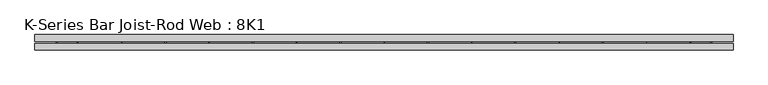
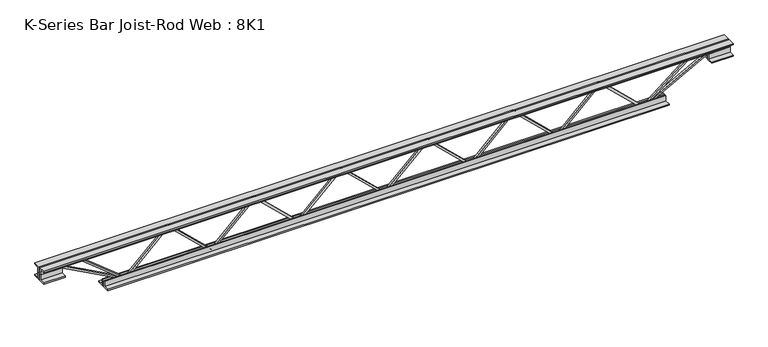
"""IFC4 building model written with IfcOpenShell, lengths in millimetres: beam geometry, K-Series Bar Joist-Rod Web : 8K1."""

import ifcopenshell
import ifcopenshell.guid

model = None  # the IFC model being written
_history = None  # IfcOwnerHistory: only IFC2X3 demands one
_inside = {}  # id of a spatial element -> (the spatial element, [elements in it])
_under = {}  # id of a project, library or spatial element -> (it, [spatial elements below it])
_declared = {}  # id of a project -> (the project, [libraries it declares])
_typed = {}  # id of a type object -> (the type object, [elements of that type])
_made_of = {}  # id of a material, layer set ... -> (it, [elements and type objects made of it])


def new_model(schema):
    """Start an empty IFC model of exactly this schema.

    Asked for "IFC4X3", IfcOpenShell would pick the latest addendum, in which some entities
    have other attributes; the version numbers below select the first issue.
    IFC2X3 requires an IfcOwnerHistory on every rooted entity: one is made here for all.
    """
    global model, _history
    if schema == "IFC4X3":
        model = ifcopenshell.file(schema_version=(4, 3, 0, 0))
    else:
        model = ifcopenshell.file(schema=schema)
    _inside.clear()
    _under.clear()
    _declared.clear()
    _typed.clear()
    _made_of.clear()
    _history = None
    if model.schema == "IFC2X3":
        org = make("IfcOrganization", Name="unknown")
        user = make(
            "IfcPersonAndOrganization",
            ThePerson=make("IfcPerson", FamilyName="unknown"),
            TheOrganization=org,
        )
        app = make(
            "IfcApplication",
            ApplicationDeveloper=org,
            Version="unknown",
            ApplicationFullName="unknown",
            ApplicationIdentifier="unknown",
        )
        _history = make(
            "IfcOwnerHistory",
            OwningUser=user,
            OwningApplication=app,
            ChangeAction="ADDED",
            CreationDate=0,
        )
    return model


def make(cls, **values):
    """One entity of the class cls with the attributes given. An attribute that is None is left unset."""
    return model.create_entity(
        cls, **{name: value for name, value in values.items() if value is not None}
    )


def rooted(cls, **values):
    """An entity with a GlobalId (a new one), such as an element, a storey or a relation."""
    return make(cls, GlobalId=ifcopenshell.guid.new(), OwnerHistory=_history, **values)


def si_unit(unit_type, name, prefix=None):
    """IfcSIUnit, for example si_unit("LENGTHUNIT", "METRE", prefix="MILLI")."""
    return make("IfcSIUnit", UnitType=unit_type, Prefix=prefix, Name=name)


def assignment(units):
    """IfcUnitAssignment: the units of a project."""
    return None if units is None else make("IfcUnitAssignment", Units=units)


def point(xyz):
    """IfcCartesianPoint."""
    return None if xyz is None else make("IfcCartesianPoint", Coordinates=xyz)


def direction(xyz):
    """IfcDirection."""
    return None if xyz is None else make("IfcDirection", DirectionRatios=xyz)


def frame(location, z_axis=None, x_axis=None):
    """IfcAxis2Placement3D, a coordinate frame: its origin and axes. An axis left out is left unset."""
    return make(
        "IfcAxis2Placement3D",
        Location=point(location),
        Axis=direction(z_axis),
        RefDirection=direction(x_axis),
    )


def origin():
    """The frame at (0, 0, 0) with its axes left unset."""
    return frame((0.0, 0.0, 0.0))


def place(relative_to, where):
    """IfcLocalPlacement: puts the frame where relative to a parent placement (None: the world)."""
    return make(
        "IfcLocalPlacement", PlacementRelTo=relative_to, RelativePlacement=where
    )


def context(
    kind, dimensions, precision=None, world=None, true_north=None, identifier=None
):
    """IfcGeometricRepresentationContext, for example the 3D "Model" context."""
    return make(
        "IfcGeometricRepresentationContext",
        ContextIdentifier=identifier,
        ContextType=kind,
        CoordinateSpaceDimension=dimensions,
        Precision=precision,
        WorldCoordinateSystem=world,
        TrueNorth=true_north,
    )


def project(units=None, contexts=None):
    """IfcProject with its units and contexts."""
    return rooted(
        "IfcProject",
        Name="project",
        RepresentationContexts=contexts,
        UnitsInContext=assignment(units),
    )


def spatial(cls, under=None, at=None, **own):
    """A site, building, storey or space (cls), placed at a placement, below another one or the project."""
    s = rooted(cls, ObjectPlacement=at, **own)
    if under is not None:
        _under.setdefault(under.id(), (under, []))[1].append(s)
    return s


def polyline(points):
    """IfcPolyline through the points."""
    return make("IfcPolyline", Points=[point(p) for p in points])


def outline(outer, holes=None, kind="AREA"):
    """IfcArbitraryClosedProfileDef: a profile drawn as a closed curve; with holes, ...WithVoids."""
    if holes is None:
        return make("IfcArbitraryClosedProfileDef", ProfileType=kind, OuterCurve=outer)
    return make(
        "IfcArbitraryProfileDefWithVoids",
        ProfileType=kind,
        OuterCurve=outer,
        InnerCurves=holes,
    )


def extrude(swept, where, along, depth):
    """IfcExtrudedAreaSolid: the profile swept, set in the frame where, extruded along a direction by depth."""
    return make(
        "IfcExtrudedAreaSolid",
        SweptArea=swept,
        Position=where,
        ExtrudedDirection=direction(along),
        Depth=depth,
    )


def shape(context_of_items, identifier, shape_type, items):
    """IfcShapeRepresentation: the items that make up one representation, for example the "Body"."""
    return make(
        "IfcShapeRepresentation",
        ContextOfItems=context_of_items,
        RepresentationIdentifier=identifier,
        RepresentationType=shape_type,
        Items=items,
    )


def source(mapping_origin, context_of_items, identifier, shape_type, items):
    """IfcRepresentationMap: a shape defined once, which mapped items show again and again."""
    return make(
        "IfcRepresentationMap",
        MappingOrigin=mapping_origin,
        MappedRepresentation=shape(context_of_items, identifier, shape_type, items),
    )


def transform(
    local_origin,
    x_axis=None,
    y_axis=None,
    z_axis=None,
    scale=None,
    scale2=None,
    scale3=None,
    uniform=True,
):
    """IfcCartesianTransformationOperator3D, or its non-uniform kind. x_axis, y_axis, z_axis: its Axis1, 2, 3."""
    if uniform:
        return make(
            "IfcCartesianTransformationOperator3D",
            Axis1=direction(x_axis),
            Axis2=direction(y_axis),
            LocalOrigin=point(local_origin),
            Scale=scale,
            Axis3=direction(z_axis),
        )
    return make(
        "IfcCartesianTransformationOperator3DnonUniform",
        Axis1=direction(x_axis),
        Axis2=direction(y_axis),
        LocalOrigin=point(local_origin),
        Scale=scale,
        Axis3=direction(z_axis),
        Scale2=scale2,
        Scale3=scale3,
    )


def mapped(mapping_source, mapping_target):
    """IfcMappedItem: shows the shape of a source again, moved by a transform."""
    return make(
        "IfcMappedItem", MappingSource=mapping_source, MappingTarget=mapping_target
    )


def made_of(thing, what):
    """Note that an element or type object is made of a material, layer set ...; save() writes the relation."""
    if what is not None:
        _made_of.setdefault(what.id(), (what, []))[1].append(thing)
    return thing


def element(
    cls,
    number,
    at=None,
    inside=None,
    cuts=None,
    type_object=None,
    material=None,
    context=None,
    identifier="Body",
    shape_type=None,
    held_by="IfcProductDefinitionShape",
    body=None,
    shapes=None,
    **own,
):
    """One element of the class cls, such as IfcWall. Its Tag is "e" and its number.

    at: its placement. inside: the storey or other place that contains it. cuts: it is an
    opening in that element (IfcRelVoidsElement). A single representation is given by context,
    identifier, shape_type and body (its items); several are given by shapes. held_by: the class
    of the entity that holds the representations. save() writes the other relations.
    """
    e = rooted(cls, Tag="e%d" % number, ObjectPlacement=at, **own)
    if body is not None:
        shapes = [shape(context, identifier, shape_type, body)]
    if shapes is not None:
        e.Representation = make(held_by, Representations=shapes)
    if inside is not None:
        _inside.setdefault(inside.id(), (inside, []))[1].append(e)
    if cuts is not None:
        rooted(
            "IfcRelVoidsElement", RelatingBuildingElement=cuts, RelatedOpeningElement=e
        )
    if type_object is not None:
        _typed.setdefault(type_object.id(), (type_object, []))[1].append(e)
    return made_of(e, material)


def aggregate(whole, parts):
    """IfcRelAggregates: a whole, such as a stair, and the parts it consists of."""
    return rooted("IfcRelAggregates", RelatingObject=whole, RelatedObjects=parts)


def save(model, path):
    """Write the relations noted so far, then the file.

    IfcRelAggregates (storeys below a building ...), IfcRelContainedInSpatialStructure (elements
    in a storey), IfcRelDefinesByType, IfcRelAssociatesMaterial and IfcRelDeclares: one each for
    every whole, place, type object, material and project.
    """
    for whole, parts in _under.values():
        aggregate(whole, parts)
    for where, things in _inside.values():
        rooted(
            "IfcRelContainedInSpatialStructure",
            RelatedElements=things,
            RelatingStructure=where,
        )
    for kind, things in _typed.values():
        rooted("IfcRelDefinesByType", RelatedObjects=things, RelatingType=kind)
    for what, things in _made_of.values():
        rooted("IfcRelAssociatesMaterial", RelatedObjects=things, RelatingMaterial=what)
    for by, libraries in _declared.values():
        rooted("IfcRelDeclares", RelatingContext=by, RelatedDefinitions=libraries)
    model.write(path)


def k_series_bar_joist_rod_web_8k1_5ba47054(model_context):
    return source(origin(), model_context, "Body", "SweptSolid", [
        extrude(outline(polyline([(-90.4875, 411.0474986), (-100.0125, 411.0474986), (-100.0125, 416.133385), (90.4875, 615.3071343), (90.4875, 617.8353616), (-100.0125, 817.0091109), (-100.0125, 822.0949973), (-90.4875, 822.0949973), (-90.4875, 820.8308836), (100.0125, 621.6571343), (100.0125, 611.4853616), (-90.4875, 412.3116123), (-90.4875, 411.0474986)])), frame((0.0, -4.7625, 0.0), z_axis=(0.0, 1.0, 0.0), x_axis=(0.0, 0.0, 1.0)), (0.0, 0.0, 1.0), 9.525),
        extrude(outline(polyline([(-90.4875, 0.0), (-100.0125, 0.0), (-100.0125, 5.0858863), (90.4875, 204.2596356), (90.4875, 206.787863), (-100.0125, 405.9616123), (-100.0125, 411.0474986), (-90.4875, 411.0474986), (-90.4875, 409.783385), (100.0125, 210.6096356), (100.0125, 200.437863), (-90.4875, 1.2641137), (-90.4875, 0.0)])), frame((0.0, -4.7625, 0.0), z_axis=(0.0, 1.0, 0.0), x_axis=(0.0, 0.0, 1.0)), (0.0, 0.0, 1.0), 9.525),
        extrude(outline(polyline([(-90.4875, -411.0474986), (-100.0125, -411.0474986), (-100.0125, -405.9616123), (90.4875, -206.787863), (90.4875, -204.2596356), (-100.0125, -5.0858863), (-100.0125, 0.0), (-90.4875, 0.0), (-90.4875, -1.2641137), (100.0125, -200.437863), (100.0125, -210.6096356), (-90.4875, -409.783385), (-90.4875, -411.0474986)])), frame((0.0, -4.7625, 0.0), z_axis=(0.0, 1.0, 0.0), x_axis=(0.0, 0.0, 1.0)), (0.0, 0.0, 1.0), 9.525),
        extrude(outline(polyline([(-90.4875, -822.0949973), (-100.0125, -822.0949973), (-100.0125, -817.0091109), (90.4875, -617.8353616), (90.4875, -615.3071343), (-100.0125, -416.133385), (-100.0125, -411.0474986), (-90.4875, -411.0474986), (-90.4875, -412.3116123), (100.0125, -611.4853616), (100.0125, -621.6571343), (-90.4875, -820.8308836), (-90.4875, -822.0949973)])), frame((0.0, -4.7625, 0.0), z_axis=(0.0, 1.0, 0.0), x_axis=(0.0, 0.0, 1.0)), (0.0, 0.0, 1.0), 9.525),
        extrude(outline(polyline([(-90.4875, 822.0949973), (-100.0125, 822.0949973), (-100.0125, 827.1808836), (90.4875, 1026.3546329), (90.4875, 1028.8828602), (-100.0125, 1228.0566096), (-100.0125, 1233.1424959), (-90.4875, 1233.1424959), (-90.4875, 1231.8783822), (100.0125, 1032.7046329), (100.0125, 1022.5328602), (-90.4875, 823.3591109), (-90.4875, 822.0949973)])), frame((0.0, -4.7625, 0.0), z_axis=(0.0, 1.0, 0.0), x_axis=(0.0, 0.0, 1.0)), (0.0, 0.0, 1.0), 9.525),
        extrude(outline(polyline([(-90.4875, -1233.1424959), (-100.0125, -1233.1424959), (-100.0125, -1228.0566096), (90.4875, -1028.8828602), (90.4875, -1026.3546329), (-100.0125, -827.1808836), (-100.0125, -822.0949973), (-90.4875, -822.0949973), (-90.4875, -823.3591109), (100.0125, -1022.5328602), (100.0125, -1032.7046329), (-90.4875, -1231.8783822), (-90.4875, -1233.1424959)])), frame((0.0, -4.7625, 0.0), z_axis=(0.0, 1.0, 0.0), x_axis=(0.0, 0.0, 1.0)), (0.0, 0.0, 1.0), 9.525),
        extrude(outline(polyline([(4.7625, 101.6), (36.5125, 101.6), (36.5125, 95.25), (11.1125, 95.25), (11.1125, 69.85), (4.7625, 69.85), (4.7625, 101.6)])), frame((-1639.5424959, 0.0, 0.0), z_axis=(1.0, 0.0, 0.0), x_axis=(0.0, 1.0, 0.0)), (0.0, 0.0, 1.0), 3279.0849918),
        extrude(outline(polyline([(-4.7625, 101.6), (-4.7625, 69.85), (-11.1125, 69.85), (-11.1125, 95.25), (-36.5125, 95.25), (-36.5125, 101.6), (-4.7625, 101.6)])), frame((-1639.5424959, 0.0, 0.0), z_axis=(1.0, 0.0, 0.0), x_axis=(0.0, 1.0, 0.0)), (0.0, 0.0, 1.0), 3279.0849918),
        extrude(outline(polyline([(-4.7625, 38.1), (-36.5125, 38.1), (-36.5125, 44.45), (-11.1125, 44.45), (-11.1125, 69.85), (-4.7625, 69.85), (-4.7625, 38.1)])), frame((-1639.5424959, 0.0, 0.0), z_axis=(1.0, 0.0, 0.0), x_axis=(0.0, 1.0, 0.0)), (0.0, 0.0, 1.0), 101.6),
        extrude(outline(polyline([(36.5125, 38.1), (4.7625, 38.1), (4.7625, 69.85), (11.1125, 69.85), (11.1125, 44.45), (36.5125, 44.45), (36.5125, 38.1)])), frame((-1639.5424959, 0.0, 0.0), z_axis=(1.0, 0.0, 0.0), x_axis=(0.0, 1.0, 0.0)), (0.0, 0.0, 1.0), 101.6),
        extrude(outline(polyline([(4.7625, 38.1), (4.7625, 69.85), (11.1125, 69.85), (11.1125, 44.45), (36.5125, 44.45), (36.5125, 38.1), (4.7625, 38.1)])), frame((1537.9424959, 0.0, 0.0), z_axis=(1.0, 0.0, 0.0), x_axis=(0.0, 1.0, 0.0)), (0.0, 0.0, 1.0), 101.6),
        extrude(outline(polyline([(-4.7625, 38.1), (-36.5125, 38.1), (-36.5125, 44.45), (-11.1125, 44.45), (-11.1125, 69.85), (-4.7625, 69.85), (-4.7625, 38.1)])), frame((1537.9424959, 0.0, 0.0), z_axis=(1.0, 0.0, 0.0), x_axis=(0.0, 1.0, 0.0)), (0.0, 0.0, 1.0), 101.6),
        extrude(outline(polyline([(4.7625, -101.6), (4.7625, -69.85), (11.1125, -69.85), (11.1125, -95.25), (36.5125, -95.25), (36.5125, -101.6), (4.7625, -101.6)])), frame((-1334.7424959, 0.0, 0.0), z_axis=(1.0, 0.0, 0.0), x_axis=(0.0, 1.0, 0.0)), (0.0, 0.0, 1.0), 2669.4849918),
        extrude(outline(polyline([(-4.7625, -101.6), (-36.5125, -101.6), (-36.5125, -95.25), (-11.1125, -95.25), (-11.1125, -69.85), (-4.7625, -69.85), (-4.7625, -101.6)])), frame((-1334.7424959, 0.0, 0.0), z_axis=(1.0, 0.0, 0.0), x_axis=(0.0, 1.0, 0.0)), (0.0, 0.0, 1.0), 2669.4849918),
        extrude(outline(polyline([(0.0, -9.525), (0.0, 0.0), (346.6425392, 0.0), (346.6425392, -9.525), (0.0, -9.525)])), frame((-1540.2107944, 4.7625, 65.662372), z_axis=(0.47628314854007997, 0.0, 0.8792919665371384), x_axis=(0.8792919665371384, 0.0, -0.47628314854007997)), (0.0, 0.0, 1.0), 9.525),
        extrude(outline(polyline([(0.0, -9.525), (0.0, 0.0), (263.6247741, 0.0), (263.6247741, -9.525), (0.0, -9.525)])), frame((-1441.6488509, 4.7625, 66.1371211), z_axis=(0.6262689102285063, 0.0, 0.7796071139241862), x_axis=(0.7796071139241862, 0.0, -0.6262689102285063)), (0.0, 0.0, 1.0), 9.525),
        extrude(outline(polyline([(0.0, -9.525), (0.0, 0.0), (346.6425392, 0.0), (346.6425392, -9.525), (0.0, -9.525)])), frame((1540.2107944, -4.7625, 65.662372), z_axis=(-0.47628314854004167, 0.0, 0.8792919665371591), x_axis=(-0.8792919665371591, 0.0, -0.47628314854004167)), (0.0, 0.0, 1.0), 9.525),
        extrude(outline(polyline([(0.0, -9.525), (0.0, 0.0), (263.6247741, 0.0), (263.6247741, -9.525), (0.0, -9.525)])), frame((1441.6488509, -4.7625, 66.1371211), z_axis=(-0.6262689102284817, 0.0, 0.779607113924206), x_axis=(-0.779607113924206, 0.0, -0.6262689102284817)), (0.0, 0.0, 1.0), 9.525),
    ])


if __name__ == "__main__":
    model = new_model("IFC4")
    model_context = context("Model", 3, world=origin())
    ifc_project = project(units=[si_unit("LENGTHUNIT", "METRE", prefix="MILLI")], contexts=[model_context])
    site = spatial("IfcSite", under=ifc_project)
    building = spatial("IfcBuilding", under=site)
    placement = place(None, origin())
    k_series_bar_joist_rod_web_8k1_shape = k_series_bar_joist_rod_web_8k1_5ba47054(model_context)
    element("IfcBeam", 1, ObjectType="K-Series Bar Joist-Rod Web : 8K1", at=placement, inside=building, context=model_context, shape_type="MappedRepresentation", body=[
        mapped(k_series_bar_joist_rod_web_8k1_shape, transform((0.0, 0.0, 0.0), x_axis=(1.0, 0.0, 0.0), y_axis=(0.0, 1.0, 0.0), z_axis=(0.0, 0.0, 1.0))),
    ])
    save(model, "model.ifc")

# Revit data of these elements
# Type "K-Series Bar Joist-Rod Web : 8K1"
#   Assembly Code = "B1010350"
#   Wt = 5.1
#   Web Thickness = 0' - 0 3/8"
#   Start Offset [instance default] = 0' - 0"
#   Start Extension [instance default] = 0' - 0"
#   Seat Length = 0' - 4"
#   Seat Depth = 0' - 2 1/2"
#   PanelArrayLength [instance default] = 21' - 4"
#   Panel [instance default] = 1' - 4"
#   End Offset [instance default] = 0' - 0"
#   End Extension [instance default] = 0' - 0"
#   End Panel = 1' - 4"
#   Cord Leg = 0' - 1 1/4"
#   Chord Thickness = 0' - 0 1/4"
#   Length [instance default] = 24' - 0"
#   Depth = 0' - 8"
#   PanelArrayNum [instance default] = 16
#   Rendering Material = none
# Element 1 (IfcBeam, "K-Series Bar Joist-Rod Web : 8K1")
#   PanelArrayLength = 8' - 1.09783"
#   Panel = 1' - 4.18297"
#   PanelArrayNum = 6
